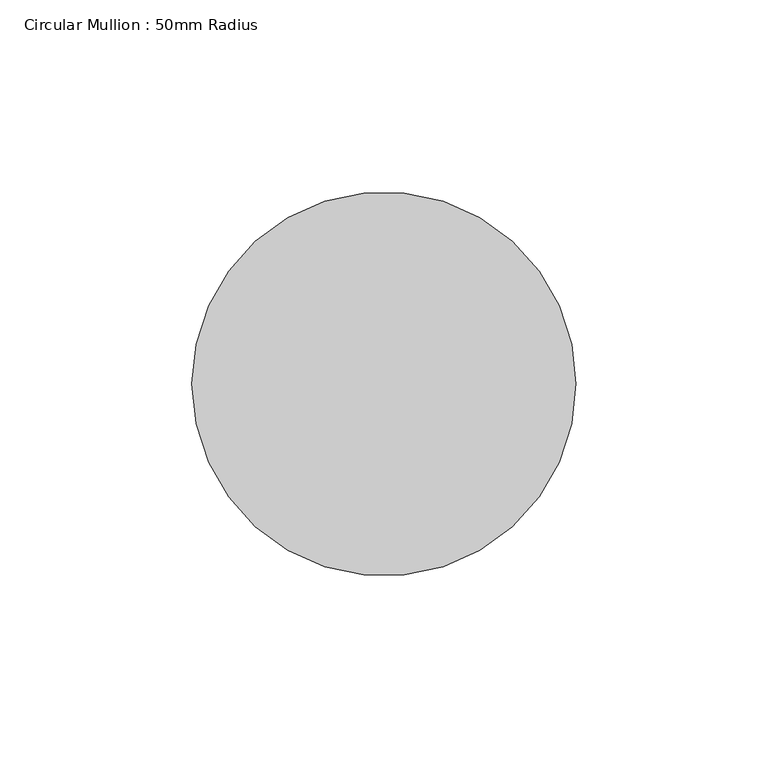
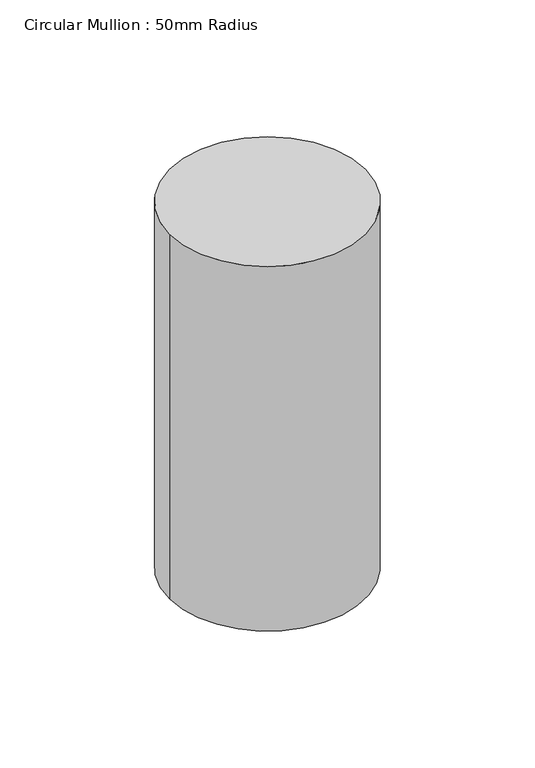
"""IFC4 building model written with IfcOpenShell, lengths in millimetres: member geometry, Circular Mullion : 50mm Radius."""

from ifc_helpers import new_model, si_unit, point, frame, origin, origin_2d, place, context, project, spatial, circle_curve, trimmed, segment, composite_curve, outline, extrude, source, transform, mapped, element, save


def circular_mullion_50mm_radius_022099a0(model_context):
    return source(origin(), model_context, "Body", "SweptSolid", [
        extrude(outline(composite_curve([segment(trimmed(circle_curve(origin_2d(), 50.0), [point((50.0, 0.0))], [point((-50.0, 0.0))], False, "CARTESIAN"), True, "CONTINUOUS"), segment(trimmed(circle_curve(origin_2d(), 50.0), [point((-50.0, 0.0))], [point((50.0, 0.0))], False, "CARTESIAN"), True, "CONTINUOUS")], self_intersect=False)), frame((0.0, 0.0, -196.7849414), z_axis=(0.0, 0.0, 1.0), x_axis=(1.0, 0.0, 0.0)), (0.0, 0.0, 1.0), 196.7849414),
    ])


if __name__ == "__main__":
    model = new_model("IFC4")
    model_context = context("Model", 3, world=origin())
    ifc_project = project(units=[si_unit("LENGTHUNIT", "METRE", prefix="MILLI")], contexts=[model_context])
    site = spatial("IfcSite", under=ifc_project)
    building = spatial("IfcBuilding", under=site)
    placement = place(None, origin())
    circular_mullion_50mm_radius_shape = circular_mullion_50mm_radius_022099a0(model_context)
    element("IfcMember", 1, ObjectType="Circular Mullion : 50mm Radius", at=placement, inside=building, context=model_context, shape_type="MappedRepresentation", body=[
        mapped(circular_mullion_50mm_radius_shape, transform((0.0, 0.0, 0.0), x_axis=(1.0, 0.0, 0.0), y_axis=(0.0, 1.0, 0.0), z_axis=(0.0, 0.0, 1.0))),
    ])
    save(model, "model.ifc")

# Revit data of these elements
# Type "Circular Mullion : 50mm Radius"
#   built-in parameter 1007350 = 0.164042 (stored number, unit not read)
# Element 1 (IfcMember, "Circular Mullion : 50mm Radius")
#   Materials on its faces: "Aluminium"
# Materials
#   "Aluminium": class "Metal", colour RGB 247 247 247, transparency 0, Description = "Aluminium 6061", Cost = 0
